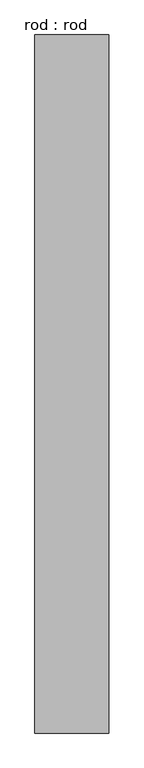
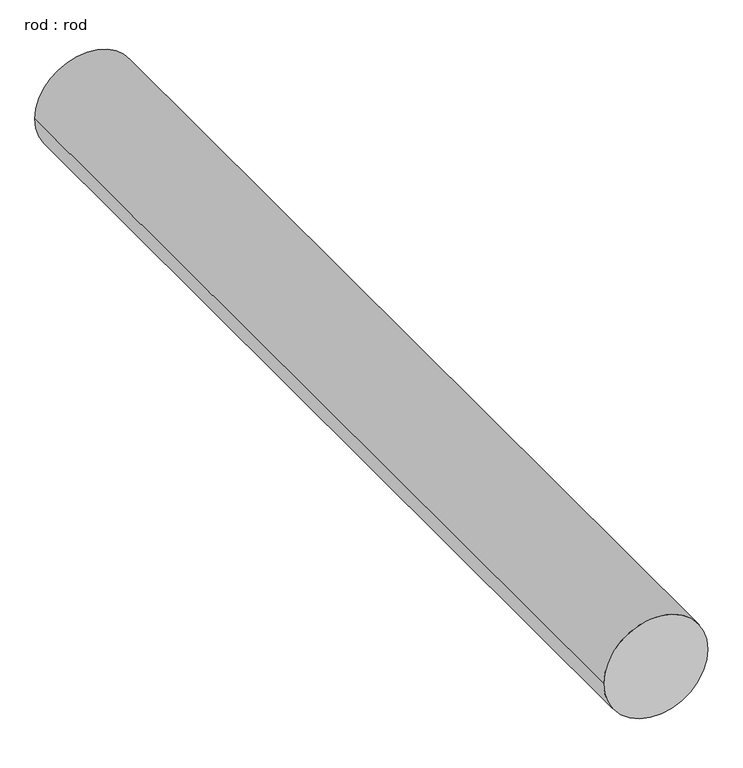
"""IFC4 building model written with IfcOpenShell, lengths in millimetres: proxy geometry, rod : rod."""

from ifc_helpers import new_model, si_unit, point, frame, frame_2d, origin, place, context, project, spatial, circle_curve, trimmed, segment, composite_curve, outline, extrude, source, transform, mapped, element, save


def rod_rod_792636d3(model_context):
    return source(origin(), model_context, "Body", "SweptSolid", [
        extrude(outline(composite_curve([segment(trimmed(circle_curve(frame_2d((0.0108462, 0.0)), 200.0), [point((0.0108462, 200.0))], [point((0.0108462, -200.0))], False, "CARTESIAN"), True, "CONTINUOUS"), segment(trimmed(circle_curve(frame_2d((0.0108462, 0.0)), 200.0), [point((0.0108462, -200.0))], [point((0.0108462, 200.0))], False, "CARTESIAN"), True, "CONTINUOUS")], self_intersect=False)), frame((0.0, 2204.4605597, 0.0), z_axis=(0.0, 1.0, 0.0), x_axis=(0.0, 0.0, 1.0)), (0.0, 0.0, 1.0), 3776.5361113),
    ])


if __name__ == "__main__":
    model = new_model("IFC4")
    model_context = context("Model", 3, world=origin())
    ifc_project = project(units=[si_unit("LENGTHUNIT", "METRE", prefix="MILLI")], contexts=[model_context])
    site = spatial("IfcSite", under=ifc_project)
    building = spatial("IfcBuilding", under=site)
    placement = place(None, origin())
    rod_rod_shape = rod_rod_792636d3(model_context)
    element("IfcBuildingElementProxy", 1, Name="rod : rod", ObjectType="rod : rod", at=placement, inside=building, context=model_context, shape_type="MappedRepresentation", body=[
        mapped(rod_rod_shape, transform((0.0, 0.0, 0.0), x_axis=(1.0, 0.0, 0.0), y_axis=(0.0, 1.0, 0.0), z_axis=(0.0, 0.0, 1.0))),
    ])
    save(model, "model.ifc")

# Revit data of these elements
# Type "rod : rod"
#   Default Elevation = 0
